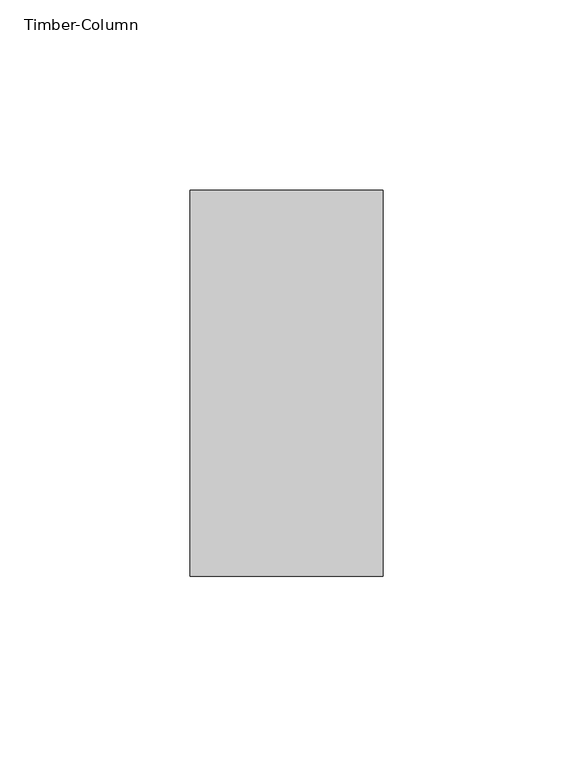
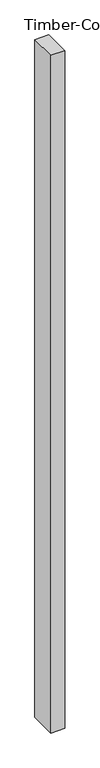
"""IFC4 building model written with IfcOpenShell, lengths in millimetres: column geometry, Timber-Column."""

from ifc_helpers import new_model, si_unit, frame, origin, place, context, project, spatial, polyline, outline, extrude, source, transform, mapped, element, save


def timber_column_c014de30(model_context):
    return source(origin(), model_context, "Body", "SweptSolid", [
        extrude(outline(polyline([(25.4, -50.8), (-25.4, -50.8), (-25.4, 50.8), (25.4, 50.8), (25.4, -50.8)])), frame((0.0, 0.0, 50.8), z_axis=(0.0, 0.0, 1.0), x_axis=(1.0, 0.0, 0.0)), (0.0, 0.0, 1.0), 2616.2),
    ])


if __name__ == "__main__":
    model = new_model("IFC4")
    model_context = context("Model", 3, world=origin())
    ifc_project = project(units=[si_unit("LENGTHUNIT", "METRE", prefix="MILLI")], contexts=[model_context])
    site = spatial("IfcSite", under=ifc_project)
    building = spatial("IfcBuilding", under=site)
    placement = place(None, origin())
    timber_column_shape = timber_column_c014de30(model_context)
    element("IfcColumn", 1, ObjectType="Timber-Column : BLDG 6241 Wall Struds 2\"x4\"", at=placement, inside=building, context=model_context, shape_type="MappedRepresentation", body=[
        mapped(timber_column_shape, transform((0.0, 0.0, 0.0), x_axis=(1.0, 0.0, 0.0), y_axis=(0.0, 1.0, 0.0), z_axis=(0.0, 0.0, 1.0))),
    ])
    save(model, "model.ifc")

# Revit data of these elements
# Type "Timber-Column : BLDG 6241 Wall Struds 2\"x4\""
#   Assembly Code = "B10"
#   A = 0.140625 SF
#   b = 0' - 2"
#   d = 0' - 4"
#   Structural Material [instance default] = Softwood, Lumber
# Element 1 (IfcColumn, "Timber-Column : BLDG 6241 Wall Struds 2\"x4\"")
#   Materials on its faces: "Softwood, Lumber"
# Materials
#   "Softwood, Lumber": class "Wood", colour RGB 223 192 134, transparency 0, Description = "Pinus Echinata", Cost = 0
